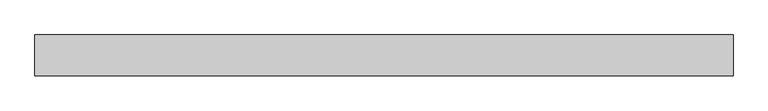
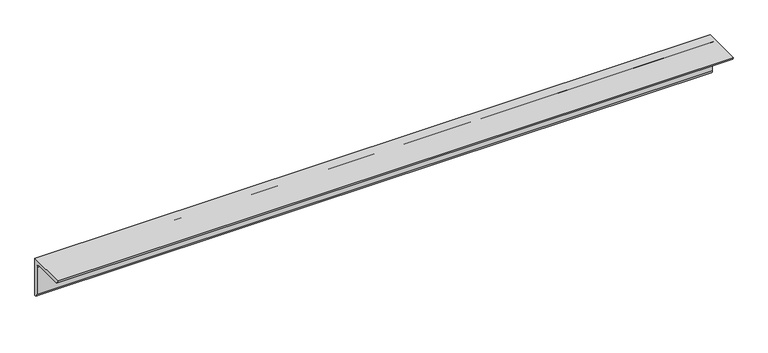
"""IFC4 building model written with IfcOpenShell, lengths in millimetres: member geometry, 0912_Steel Framing_L-KSD3502 : H_SB_AR_S03_L-130x130x12_HBR3."""

from ifc_helpers import new_model, si_unit, point, frame, frame_2d, origin, place, context, project, spatial, polyline, circle_curve, trimmed, segment, composite_curve, outline, extrude, source, transform, mapped, element, save


def member_39229cb8(model_context):
    return source(origin(), model_context, "Body", "SweptSolid", [
        extrude(outline(composite_curve([segment(polyline([(36.4, 36.4), (36.4, -93.6)]), True, "CONTINUOUS"), segment(trimmed(circle_curve(frame_2d((36.4, -81.6)), 12.0), [point((36.4, -93.6))], [point((24.4, -81.6))], False, "CARTESIAN"), True, "CONTINUOUS"), segment(polyline([(24.4, -81.6), (24.4, 12.4)]), True, "CONTINUOUS"), segment(trimmed(circle_curve(frame_2d((12.4, 12.4)), 12.0), [point((24.4, 12.4))], [point((12.4, 24.4))], True, "CARTESIAN"), True, "CONTINUOUS"), segment(polyline([(12.4, 24.4), (-81.6, 24.4)]), True, "CONTINUOUS"), segment(trimmed(circle_curve(frame_2d((-81.6, 36.4)), 12.0), [point((-81.6, 24.4))], [point((-93.6, 36.4))], False, "CARTESIAN"), True, "CONTINUOUS"), segment(polyline([(-93.6, 36.4), (36.4, 36.4)]), True, "CONTINUOUS")], self_intersect=False)), frame((-1213.4037947, 0.0, 0.0), z_axis=(1.0, 0.0, 0.0), x_axis=(0.0, 1.0, 0.0)), (0.0, 0.0, 1.0), 2227.2361155),
    ])


if __name__ == "__main__":
    model = new_model("IFC4")
    model_context = context("Model", 3, world=origin())
    ifc_project = project(units=[si_unit("LENGTHUNIT", "METRE", prefix="MILLI")], contexts=[model_context])
    site = spatial("IfcSite", under=ifc_project)
    building = spatial("IfcBuilding", under=site)
    placement = place(None, origin())
    member_shape = member_39229cb8(model_context)
    element("IfcMember", 1, ObjectType="0912_Steel Framing_L-KSD3502 : H_SB_AR_S03_L-130x130x12_HBR3", at=placement, inside=building, context=model_context, shape_type="MappedRepresentation", body=[
        mapped(member_shape, transform((0.0, 0.0, 0.0), x_axis=(1.0, 0.0, 0.0), y_axis=(0.0, 1.0, 0.0), z_axis=(0.0, 0.0, 1.0))),
    ])
    save(model, "model.ifc")

# Revit data of these elements
# Type "0912_Steel Framing_L-KSD3502 : H_SB_AR_S03_L-130x130x12_HBR3"
#   k = 25 mm
#   Perimeter = 0.52 m²/m
#   Nominal Weight = 23.40 kgf/m
#   Length [instance default] = 1000 mm
#   b = 130 mm
#   d = 130 mm
#   t = 12 mm
#   x = 36.4 mm
#   y = 36.4 mm
#   A = 2976.00 m²
#   Structural Material [instance default] = Steel, 45-345
# Element 1 (IfcMember, "0912_Steel Framing_L-KSD3502 : H_SB_AR_S03_L-130x130x12_HBR3")
#   Structural Material = Steel ASTM A36
#   Materials on its faces: "Steel ASTM A36"
# Materials
#   "Steel, 45-345": class "Metal", colour RGB 189 187 185, transparency 0, Description = "Steel 345 MPa", Cost = 0
#   "Steel ASTM A36": class "Metal", colour RGB 199 199 199, transparency 0, Description = "Structural steel, ASTM A36 Grade B, mill finish", Cost = 0
